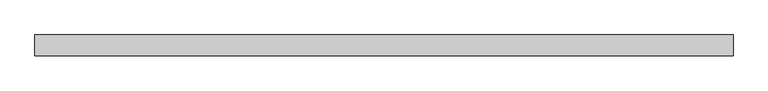
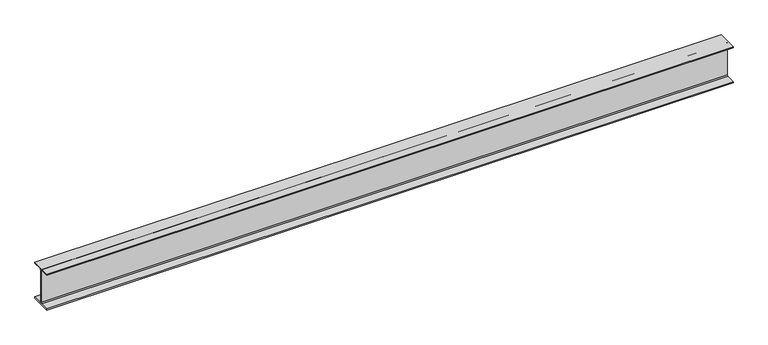
"""IFC4 building model written with IfcOpenShell, lengths in millimetres: beam geometry, Old_Steel Beam_H-KSD3502 : H_SB_ASB_H-200×200x8x12."""

from ifc_helpers import new_model, si_unit, point, frame, frame_2d, origin, place, context, project, spatial, polyline, circle_curve, trimmed, segment, composite_curve, outline, extrude, source, transform, mapped, element, save


def beam_4a306e14(model_context):
    return source(origin(), model_context, "Body", "SweptSolid", [
        extrude(outline(composite_curve([segment(polyline([(82.5, -141.5), (82.5, -151.7), (-82.5, -151.7), (-82.5, -141.5), (-11.9, -141.5)]), True, "CONTINUOUS"), segment(trimmed(circle_curve(frame_2d((-11.9, -132.6)), 8.9), [point((-11.9, -141.5))], [point((-3.0, -132.6))], True, "CARTESIAN"), True, "CONTINUOUS"), segment(polyline([(-3.0, -132.6), (-3.0, 132.6)]), True, "CONTINUOUS"), segment(trimmed(circle_curve(frame_2d((-11.9, 132.6)), 8.9), [point((-3.0, 132.6))], [point((-11.9, 141.5))], True, "CARTESIAN"), True, "CONTINUOUS"), segment(polyline([(-11.9, 141.5), (-82.5, 141.5), (-82.5, 151.7), (82.5, 151.7), (82.5, 141.5), (11.9, 141.5)]), True, "CONTINUOUS"), segment(trimmed(circle_curve(frame_2d((11.9, 132.6)), 8.9), [point((11.9, 141.5))], [point((3.0, 132.6))], True, "CARTESIAN"), True, "CONTINUOUS"), segment(polyline([(3.0, 132.6), (3.0, -132.6)]), True, "CONTINUOUS"), segment(trimmed(circle_curve(frame_2d((11.9, -132.6)), 8.9), [point((3.0, -132.6))], [point((11.9, -141.5))], True, "CARTESIAN"), True, "CONTINUOUS"), segment(polyline([(11.9, -141.5), (82.5, -141.5)]), True, "CONTINUOUS")], self_intersect=False)), frame((-2547.7430875, 0.0, 0.0), z_axis=(1.0, 0.0, 0.0), x_axis=(0.0, 1.0, 0.0)), (0.0, 0.0, 1.0), 5469.6621901),
    ])


if __name__ == "__main__":
    model = new_model("IFC4")
    model_context = context("Model", 3, world=origin())
    ifc_project = project(units=[si_unit("LENGTHUNIT", "METRE", prefix="MILLI")], contexts=[model_context])
    site = spatial("IfcSite", under=ifc_project)
    building = spatial("IfcBuilding", under=site)
    placement = place(None, origin())
    beam_shape = beam_4a306e14(model_context)
    element("IfcBeam", 1, ObjectType="Old_Steel Beam_H-KSD3502 : H_SB_ASB_H-200×200x8x12", at=placement, inside=building, context=model_context, shape_type="MappedRepresentation", body=[
        mapped(beam_shape, transform((0.0, 0.0, 0.0), x_axis=(1.0, 0.0, 0.0), y_axis=(0.0, 1.0, 0.0), z_axis=(0.0, 0.0, 1.0))),
    ])
    save(model, "model.ifc")

# Revit data of these elements
# Type "Old_Steel Beam_H-KSD3502 : H_SB_ASB_H-200×200x8x12"
#   Width = 20.0 cm
#   Web Thickness = 0.8 cm
#   Web Fillet = 1.3 cm
#   Warping Constant = 141376.0 cm⁶
#   Torsional Moment of Inertia = 26.2485 cm⁴
#   Torsional Modulus = 1.0 cm³
#   Section Area = 63.53 cm²
#   Plastic Modulus weak axis = 244.0 cm³
#   Plastic Modulus strong axis = 525.0 cm³
#   Perimeter = 1.16 m²/m
#   Nominal Weight = 49.90 kgf/m
#   Moment of Inertia weak axis = 1600.00 cm⁴
#   Moment of Inertia strong axis = 4720.00 cm⁴
#   Height = 20.0 cm
#   Flange Thickness = 1.2 cm
#   Elastic Modulus weak axis = 160.0 cm³
#   Elastic Modulus strong axis = 472.0 cm³
#   Centroid Vertical = 10.0 cm
#   Centroid Horizontal = 10.0 cm
#   Length [instance default] = 1.5240 m
#   Structural Material [instance default] = Steel, 45-345
#   Assembly Code = ""
# Element 1 (IfcBeam, "Old_Steel Beam_H-KSD3502 : H_SB_ASB_H-200×200x8x12")
#   Structural Material = none
# Materials
#   "Steel, 45-345": class "Metal", colour RGB 189 187 185, transparency 0, Description = "Steel 345 MPa", Cost = 0
